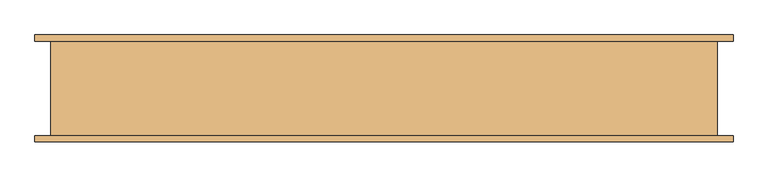
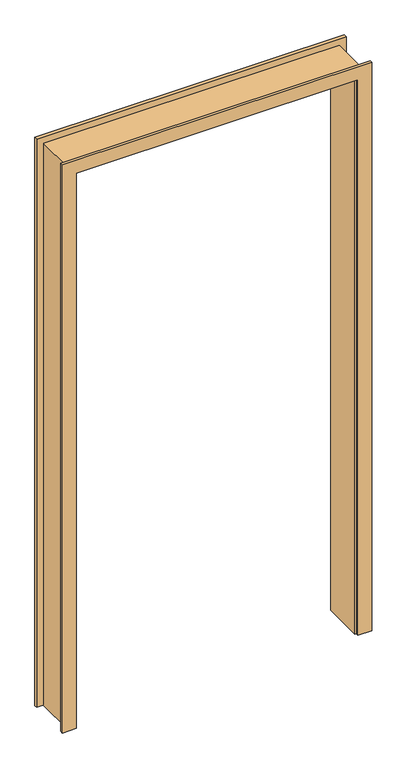
"""IFC4 building model written with IfcOpenShell, lengths in millimetres: door geometry, porta multiplas_growarq : abertura vão livre 100 cm_growarq."""

import ifcopenshell
import ifcopenshell.guid

model = None  # the IFC model being written
_history = None  # IfcOwnerHistory: only IFC2X3 demands one
_inside = {}  # id of a spatial element -> (the spatial element, [elements in it])
_under = {}  # id of a project, library or spatial element -> (it, [spatial elements below it])
_declared = {}  # id of a project -> (the project, [libraries it declares])
_typed = {}  # id of a type object -> (the type object, [elements of that type])
_made_of = {}  # id of a material, layer set ... -> (it, [elements and type objects made of it])


def new_model(schema):
    """Start an empty IFC model of exactly this schema.

    Asked for "IFC4X3", IfcOpenShell would pick the latest addendum, in which some entities
    have other attributes; the version numbers below select the first issue.
    IFC2X3 requires an IfcOwnerHistory on every rooted entity: one is made here for all.
    """
    global model, _history
    if schema == "IFC4X3":
        model = ifcopenshell.file(schema_version=(4, 3, 0, 0))
    else:
        model = ifcopenshell.file(schema=schema)
    _inside.clear()
    _under.clear()
    _declared.clear()
    _typed.clear()
    _made_of.clear()
    _history = None
    if model.schema == "IFC2X3":
        org = make("IfcOrganization", Name="unknown")
        user = make(
            "IfcPersonAndOrganization",
            ThePerson=make("IfcPerson", FamilyName="unknown"),
            TheOrganization=org,
        )
        app = make(
            "IfcApplication",
            ApplicationDeveloper=org,
            Version="unknown",
            ApplicationFullName="unknown",
            ApplicationIdentifier="unknown",
        )
        _history = make(
            "IfcOwnerHistory",
            OwningUser=user,
            OwningApplication=app,
            ChangeAction="ADDED",
            CreationDate=0,
        )
    return model


def make(cls, **values):
    """One entity of the class cls with the attributes given. An attribute that is None is left unset."""
    return model.create_entity(
        cls, **{name: value for name, value in values.items() if value is not None}
    )


def rooted(cls, **values):
    """An entity with a GlobalId (a new one), such as an element, a storey or a relation."""
    return make(cls, GlobalId=ifcopenshell.guid.new(), OwnerHistory=_history, **values)


def si_unit(unit_type, name, prefix=None):
    """IfcSIUnit, for example si_unit("LENGTHUNIT", "METRE", prefix="MILLI")."""
    return make("IfcSIUnit", UnitType=unit_type, Prefix=prefix, Name=name)


def assignment(units):
    """IfcUnitAssignment: the units of a project."""
    return None if units is None else make("IfcUnitAssignment", Units=units)


def point(xyz):
    """IfcCartesianPoint."""
    return None if xyz is None else make("IfcCartesianPoint", Coordinates=xyz)


def direction(xyz):
    """IfcDirection."""
    return None if xyz is None else make("IfcDirection", DirectionRatios=xyz)


def frame(location, z_axis=None, x_axis=None):
    """IfcAxis2Placement3D, a coordinate frame: its origin and axes. An axis left out is left unset."""
    return make(
        "IfcAxis2Placement3D",
        Location=point(location),
        Axis=direction(z_axis),
        RefDirection=direction(x_axis),
    )


def origin():
    """The frame at (0, 0, 0) with its axes left unset."""
    return frame((0.0, 0.0, 0.0))


def place(relative_to, where):
    """IfcLocalPlacement: puts the frame where relative to a parent placement (None: the world)."""
    return make(
        "IfcLocalPlacement", PlacementRelTo=relative_to, RelativePlacement=where
    )


def context(
    kind, dimensions, precision=None, world=None, true_north=None, identifier=None
):
    """IfcGeometricRepresentationContext, for example the 3D "Model" context."""
    return make(
        "IfcGeometricRepresentationContext",
        ContextIdentifier=identifier,
        ContextType=kind,
        CoordinateSpaceDimension=dimensions,
        Precision=precision,
        WorldCoordinateSystem=world,
        TrueNorth=true_north,
    )


def project(units=None, contexts=None):
    """IfcProject with its units and contexts."""
    return rooted(
        "IfcProject",
        Name="project",
        RepresentationContexts=contexts,
        UnitsInContext=assignment(units),
    )


def spatial(cls, under=None, at=None, **own):
    """A site, building, storey or space (cls), placed at a placement, below another one or the project."""
    s = rooted(cls, ObjectPlacement=at, **own)
    if under is not None:
        _under.setdefault(under.id(), (under, []))[1].append(s)
    return s


def polyline(points):
    """IfcPolyline through the points."""
    return make("IfcPolyline", Points=[point(p) for p in points])


def outline(outer, holes=None, kind="AREA"):
    """IfcArbitraryClosedProfileDef: a profile drawn as a closed curve; with holes, ...WithVoids."""
    if holes is None:
        return make("IfcArbitraryClosedProfileDef", ProfileType=kind, OuterCurve=outer)
    return make(
        "IfcArbitraryProfileDefWithVoids",
        ProfileType=kind,
        OuterCurve=outer,
        InnerCurves=holes,
    )


def extrude(swept, where, along, depth):
    """IfcExtrudedAreaSolid: the profile swept, set in the frame where, extruded along a direction by depth."""
    return make(
        "IfcExtrudedAreaSolid",
        SweptArea=swept,
        Position=where,
        ExtrudedDirection=direction(along),
        Depth=depth,
    )


def shape(context_of_items, identifier, shape_type, items):
    """IfcShapeRepresentation: the items that make up one representation, for example the "Body"."""
    return make(
        "IfcShapeRepresentation",
        ContextOfItems=context_of_items,
        RepresentationIdentifier=identifier,
        RepresentationType=shape_type,
        Items=items,
    )


def source(mapping_origin, context_of_items, identifier, shape_type, items):
    """IfcRepresentationMap: a shape defined once, which mapped items show again and again."""
    return make(
        "IfcRepresentationMap",
        MappingOrigin=mapping_origin,
        MappedRepresentation=shape(context_of_items, identifier, shape_type, items),
    )


def transform(
    local_origin,
    x_axis=None,
    y_axis=None,
    z_axis=None,
    scale=None,
    scale2=None,
    scale3=None,
    uniform=True,
):
    """IfcCartesianTransformationOperator3D, or its non-uniform kind. x_axis, y_axis, z_axis: its Axis1, 2, 3."""
    if uniform:
        return make(
            "IfcCartesianTransformationOperator3D",
            Axis1=direction(x_axis),
            Axis2=direction(y_axis),
            LocalOrigin=point(local_origin),
            Scale=scale,
            Axis3=direction(z_axis),
        )
    return make(
        "IfcCartesianTransformationOperator3DnonUniform",
        Axis1=direction(x_axis),
        Axis2=direction(y_axis),
        LocalOrigin=point(local_origin),
        Scale=scale,
        Axis3=direction(z_axis),
        Scale2=scale2,
        Scale3=scale3,
    )


def mapped(mapping_source, mapping_target):
    """IfcMappedItem: shows the shape of a source again, moved by a transform."""
    return make(
        "IfcMappedItem", MappingSource=mapping_source, MappingTarget=mapping_target
    )


def made_of(thing, what):
    """Note that an element or type object is made of a material, layer set ...; save() writes the relation."""
    if what is not None:
        _made_of.setdefault(what.id(), (what, []))[1].append(thing)
    return thing


def element(
    cls,
    number,
    at=None,
    inside=None,
    cuts=None,
    type_object=None,
    material=None,
    context=None,
    identifier="Body",
    shape_type=None,
    held_by="IfcProductDefinitionShape",
    body=None,
    shapes=None,
    **own,
):
    """One element of the class cls, such as IfcWall. Its Tag is "e" and its number.

    at: its placement. inside: the storey or other place that contains it. cuts: it is an
    opening in that element (IfcRelVoidsElement). A single representation is given by context,
    identifier, shape_type and body (its items); several are given by shapes. held_by: the class
    of the entity that holds the representations. save() writes the other relations.
    """
    e = rooted(cls, Tag="e%d" % number, ObjectPlacement=at, **own)
    if body is not None:
        shapes = [shape(context, identifier, shape_type, body)]
    if shapes is not None:
        e.Representation = make(held_by, Representations=shapes)
    if inside is not None:
        _inside.setdefault(inside.id(), (inside, []))[1].append(e)
    if cuts is not None:
        rooted(
            "IfcRelVoidsElement", RelatingBuildingElement=cuts, RelatedOpeningElement=e
        )
    if type_object is not None:
        _typed.setdefault(type_object.id(), (type_object, []))[1].append(e)
    return made_of(e, material)


def aggregate(whole, parts):
    """IfcRelAggregates: a whole, such as a stair, and the parts it consists of."""
    return rooted("IfcRelAggregates", RelatingObject=whole, RelatedObjects=parts)


def save(model, path):
    """Write the relations noted so far, then the file.

    IfcRelAggregates (storeys below a building ...), IfcRelContainedInSpatialStructure (elements
    in a storey), IfcRelDefinesByType, IfcRelAssociatesMaterial and IfcRelDeclares: one each for
    every whole, place, type object, material and project.
    """
    for whole, parts in _under.values():
        aggregate(whole, parts)
    for where, things in _inside.values():
        rooted(
            "IfcRelContainedInSpatialStructure",
            RelatedElements=things,
            RelatingStructure=where,
        )
    for kind, things in _typed.values():
        rooted("IfcRelDefinesByType", RelatedObjects=things, RelatingType=kind)
    for what, things in _made_of.values():
        rooted("IfcRelAssociatesMaterial", RelatedObjects=things, RelatingMaterial=what)
    for by, libraries in _declared.values():
        rooted("IfcRelDeclares", RelatingContext=by, RelatedDefinitions=libraries)
    model.write(path)


def door_2acfe54f(model_context):
    return source(origin(), model_context, "Body", "SweptSolid", [
        extrude(outline(polyline([(0.0, 500.0), (0.0, 530.0), (2130.0, 530.0), (2130.0, -530.0), (0.0, -530.0), (0.0, -500.0), (2100.0, -500.0), (2100.0, 500.0), (0.0, 500.0)])), frame((0.0, -75.0, 0.0), z_axis=(0.0, 1.0, 0.0), x_axis=(0.0, 0.0, 1.0)), (0.0, 0.0, 1.0), 150.0),
        extrude(outline(polyline([(2155.0, -555.0), (0.0, -555.0), (0.0, -505.0), (2105.0, -505.0), (2105.0, 505.0), (0.0, 505.0), (0.0, 555.0), (2155.0, 555.0), (2155.0, -555.0)])), frame((0.0, -85.0, 0.0), z_axis=(0.0, 1.0, 0.0), x_axis=(0.0, 0.0, 1.0)), (0.0, 0.0, 1.0), 10.0),
        extrude(outline(polyline([(2105.0, 505.0), (0.0, 505.0), (0.0, 555.0), (2155.0, 555.0), (2155.0, -555.0), (0.0, -555.0), (0.0, -505.0), (2105.0, -505.0), (2105.0, 505.0)])), frame((0.0, 75.0, 0.0), z_axis=(0.0, 1.0, 0.0), x_axis=(0.0, 0.0, 1.0)), (0.0, 0.0, 1.0), 10.0),
    ])


if __name__ == "__main__":
    model = new_model("IFC4")
    model_context = context("Model", 3, world=origin())
    ifc_project = project(units=[si_unit("LENGTHUNIT", "METRE", prefix="MILLI")], contexts=[model_context])
    site = spatial("IfcSite", under=ifc_project)
    building = spatial("IfcBuilding", under=site)
    placement = place(None, origin())
    door_shape = door_2acfe54f(model_context)
    element("IfcDoor", 1, ObjectType="porta multiplas_growarq : abertura vão livre 100 cm_growarq", at=placement, inside=building, context=model_context, shape_type="MappedRepresentation", body=[
        mapped(door_shape, transform((0.0, 0.0, 0.0), x_axis=(1.0, 0.0, 0.0), y_axis=(0.0, 1.0, 0.0), z_axis=(0.0, 0.0, 1.0))),
    ])
    save(model, "model.ifc")

# Revit data of these elements
# Type "porta multiplas_growarq : abertura vão livre 100 cm_growarq"
#   Type Mark = "A01"
#   Description = "Porta de Madeira com uma folha de abrir"
#   Analytic Construction = "<None>"
#   Rough Width = 1060 mm
#   Largura Guarnição = 50 mm
#   Espessura Guarnição = 10 mm
#   Thickness = 30 mm
#   Rough Height = 2130 mm
#   Marco = 30 mm
#   Largura Folha Eixo = 796 mm
#   Height = 2100 mm
#   Width = 1000 mm
#   Largura Folha = 996 mm
#   Eixo = 200 mm
#   Altura Folha = 2098 mm
#   Abertura correr [instance default] = 200 mm
#   Abertura [instance default] = 0.00°
#   Simples = no
#   Guarnição = yes
#   Eixo Folha = no
#   Dupla = no
#   Correr = no
#   Material = .alumínio preto_growarq
#   Function = (empty or 0)
#   Wall Closure = (empty or 0)
# Element 1 (IfcDoor, "porta multiplas_growarq : abertura vão livre 100 cm_growarq")
#   Materials on its faces: ".alumínio preto_growarq"
# Materials
#   ".alumínio preto_growarq": class "Metal", colour RGB 30 30 30, transparency 0.01, Comments = ".Enviar detalhamento das esquadrias para ter orçamento preciso", Description = "Alumínio acetinado preto", Cost = 0
